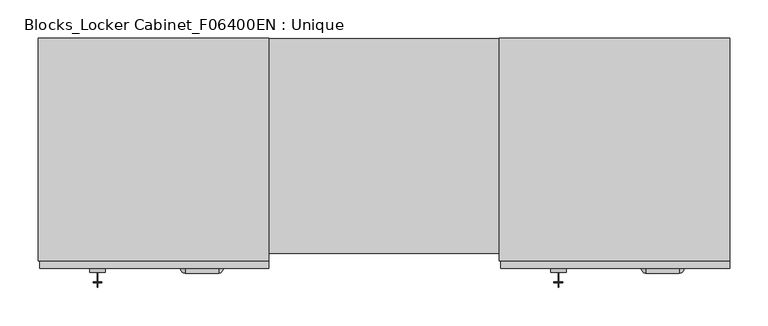
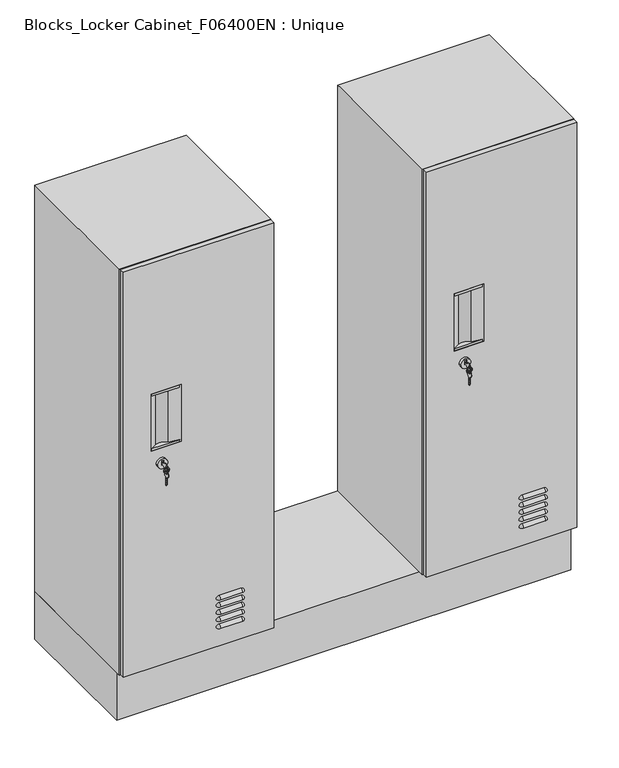
"""IFC4 building model written with IfcOpenShell, lengths in millimetres: furniture geometry, Blocks_Locker Cabinet_F06400EN : Unique."""

from ifc_helpers import new_model, si_unit, point, frame, frame_2d, origin, origin_with_axes, place, context, project, spatial, polyline, circle_curve, ellipse_curve, trimmed, segment, composite_curve, outline, extrude, faceted_brep, source, transform, mapped, element, save
from ifc_brep_helpers import plane_surface, cylinder_surface, revolved_surface, advanced_brep


def blocks_locker_cabinet_f06400en_unique_45afab01(model_context):
    return source(origin(), model_context, "Body", "SolidModel", [
        advanced_brep(
        [(217.0, -12.5, 525.0), (237.0, -12.5, 525.0), (228.8411805, -12.5, 532.0962926), (228.8411805, -12.5, 522.8618188), (225.1588195, -12.5, 522.8618188), (225.1588195, -12.5, 532.0962926), (217.0, -7.5, 525.0), (237.0, -7.5, 525.0), (217.0, -10.7450625, 525.0), (237.0, -10.7450625, 525.0), (228.8411805, -10.7450625, 532.0962926), (228.8411805, -10.7450625, 522.8618188), (225.1588195, -10.7450625, 522.8618188), (225.1588195, -10.7450625, 532.0962926)],
        [
            (0, 1, circle_curve(frame((227.0, -12.5, 525.0), z_axis=(0.0, -1.0, 0.0), x_axis=(1.0, 0.0, 0.0)), 10.0)),
            (1, 0, circle_curve(frame((227.0, -12.5, 525.0), z_axis=(0.0, -1.0, 0.0), x_axis=(1.0, 0.0, 0.0)), 10.0)),
            (2, 3),
            (3, 4),
            (4, 5),
            (5, 2),
            (6, 7, circle_curve(frame((227.0, -7.5, 525.0), z_axis=(0.0, 1.0, 0.0), x_axis=(1.0, 0.0, 0.0)), 10.0)),
            (7, 6, circle_curve(frame((227.0, -7.5, 525.0), z_axis=(0.0, 1.0, 0.0), x_axis=(1.0, 0.0, 0.0)), 10.0)),
            (0, 8),
            (8, 6),
            (7, 9),
            (9, 1),
            (2, 10),
            (10, 11),
            (11, 3),
            (11, 12),
            (12, 4),
            (12, 13),
            (13, 5),
            (13, 10),
        ],
        [
            plane_surface(frame((237.0, -12.5, 525.0), z_axis=(0.0, -1.0, 0.0), x_axis=(0.0, 0.0, 1.0))),
            plane_surface(frame((237.0, -7.5, 525.0), z_axis=(0.0, 1.0, 0.0), x_axis=(0.0, 0.0, -1.0))),
            cylinder_surface(frame((227.0, -7.5, 525.0), z_axis=(0.0, -1.0, 0.0), x_axis=(1.0, 0.0, 0.0)), 10.0),
            plane_surface(frame((228.8411805, -12.5, 532.0962926), z_axis=(-1.0, 0.0, 0.0), x_axis=(0.0, 1.0, 0.0))),
            plane_surface(frame((228.8411805, -12.5, 522.8618188), z_axis=(0.0, 0.0, 1.0), x_axis=(0.0, 1.0, 0.0))),
            plane_surface(frame((225.1588195, -12.5, 522.8618188), z_axis=(1.0, 0.0, 0.0), x_axis=(0.0, 1.0, 0.0))),
            plane_surface(frame((225.1588195, -12.5, 532.0962926), z_axis=(0.0, 0.0, -1.0), x_axis=(0.0, 1.0, 0.0))),
            plane_surface(frame((237.0, -10.7450625, 525.0), z_axis=(0.0, -1.0, 0.0), x_axis=(0.0, 0.0, 1.0))),
        ],
        [
            (0, [[1, 2], [3, 4, 5, 6]]),
            (1, [[7, 8]]),
            (2, [[-1, 9, 10, -8, 11, 12]]),
            (2, [[-2, -12, -11, -7, -10, -9]]),
            (3, [[-3, 13, 14, 15]]),
            (4, [[-4, -15, 16, 17]]),
            (5, [[-5, -17, 18, 19]]),
            (6, [[-6, -19, 20, -13]]),
            (7, [[-14, -20, -18, -16]]),
        ],
    ),
        extrude(outline(composite_curve([segment(trimmed(circle_curve(frame_2d((-23.0067332, 525.0)), 6.5414185), [point((-16.8246351, 522.8618188))], [point((-17.0336838, 527.6669902))], False, "CARTESIAN"), True, "CONTINUOUS"), segment(polyline([(-17.0336838, 527.6669902), (-10.7450625, 527.6669902), (-10.7450625, 522.8618188), (-12.0321832, 522.8618188)]), True, "CONTINUOUS"), segment(trimmed(circle_curve(frame_2d((-12.908516, 522.8618188)), 0.8763328), [point((-12.0321832, 522.8618188))], [point((-13.7848488, 522.8618188))], True, "CARTESIAN"), True, "CONTINUOUS"), segment(polyline([(-13.7848488, 522.8618188), (-16.8246351, 522.8618188)]), True, "CONTINUOUS")], self_intersect=False), holes=[composite_curve([segment(trimmed(circle_curve(frame_2d((-25.6281997, 525.0)), 1.688217), [point((-27.3164167, 525.0))], [point((-23.9399827, 525.0))], True, "CARTESIAN"), True, "CONTINUOUS"), segment(trimmed(circle_curve(frame_2d((-25.6281997, 525.0)), 1.688217), [point((-23.9399827, 525.0))], [point((-27.3164167, 525.0))], True, "CARTESIAN"), True, "CONTINUOUS")], self_intersect=False)]), frame((226.5956922, 0.0, 0.0), z_axis=(1.0, 0.0, 0.0), x_axis=(0.0, 1.0, 0.0)), (0.0, 0.0, 1.0), 0.9157402),
        extrude(outline(composite_curve([segment(trimmed(circle_curve(frame_2d((-25.6743188, 510.9839856)), 6.5414185), [point((-27.8125, 504.8018875))], [point((-24.2573286, 504.5978839))], False, "CARTESIAN"), True, "CONTINUOUS"), segment(polyline([(-24.2573286, 504.5978839), (-24.2573286, 487.7095301), (-25.9613419, 487.7095301), (-27.8125, 490.3532579), (-27.8125, 492.0094356)]), True, "CONTINUOUS"), segment(trimmed(circle_curve(frame_2d((-27.8125, 492.8857684)), 0.8763328), [point((-27.8125, 492.0094356))], [point((-27.8125, 493.7621012))], True, "CARTESIAN"), True, "CONTINUOUS"), segment(polyline([(-27.8125, 493.7621012), (-27.8125, 496.0094356)]), True, "CONTINUOUS"), segment(trimmed(circle_curve(frame_2d((-27.8125, 496.8857684)), 0.8763328), [point((-27.8125, 496.0094356))], [point((-27.8125, 497.7621012))], True, "CARTESIAN"), True, "CONTINUOUS"), segment(polyline([(-27.8125, 497.7621012), (-27.8125, 500.0094356)]), True, "CONTINUOUS"), segment(trimmed(circle_curve(frame_2d((-27.8125, 500.8857684)), 0.8763328), [point((-27.8125, 500.0094356))], [point((-27.8125, 501.7621012))], True, "CARTESIAN"), True, "CONTINUOUS"), segment(polyline([(-27.8125, 501.7621012), (-27.8125, 504.8018875)]), True, "CONTINUOUS")], self_intersect=False), holes=[composite_curve([segment(trimmed(circle_curve(frame_2d((-25.6743188, 513.6054521)), 1.688217), [point((-25.6743188, 515.2936691))], [point((-25.6743188, 511.9172351))], True, "CARTESIAN"), True, "CONTINUOUS"), segment(trimmed(circle_curve(frame_2d((-25.6743188, 513.6054521)), 1.688217), [point((-25.6743188, 511.9172351))], [point((-25.6743188, 515.2936691))], True, "CARTESIAN"), True, "CONTINUOUS")], self_intersect=False)]), frame((226.5956922, 0.0, 0.0), z_axis=(1.0, 0.0, 0.0), x_axis=(0.0, 1.0, 0.0)), (0.0, 0.0, 1.0), 0.9157402),
        advanced_brep(
        [(231.2, -25.663019, 519.4000012), (222.8, -25.663019, 519.4000012), (221.2, -25.663019, 519.4000012), (232.8, -25.663019, 519.4000012)],
        [
            (0, 1, circle_curve(frame((227.0, -25.663019, 519.4000012), z_axis=(0.0, 1.0, 0.0), x_axis=(-1.0, 0.0, 0.0)), 4.2)),
            (1, 2, circle_curve(frame((222.0, -25.663019, 519.4000012), z_axis=(0.0, 0.0, -1.0), x_axis=(1.0, 0.0, 0.0)), 0.8)),
            (2, 3, circle_curve(frame((227.0, -25.663019, 519.4000012), z_axis=(0.0, -1.0, 0.0), x_axis=(-1.0, 0.0, 0.0)), 5.8)),
            (3, 0, circle_curve(frame((232.0, -25.663019, 519.4000012), z_axis=(0.0, 0.0, -1.0), x_axis=(-1.0, 0.0, 0.0)), 0.8)),
            (2, 1, circle_curve(frame((222.0, -25.663019, 519.4000012), z_axis=(0.0, 0.0, -1.0), x_axis=(1.0, 0.0, 0.0)), 0.8)),
            (0, 3, circle_curve(frame((232.0, -25.663019, 519.4000012), z_axis=(0.0, 0.0, -1.0), x_axis=(-1.0, 0.0, 0.0)), 0.8)),
            (1, 0, circle_curve(frame((227.0, -25.663019, 519.4000012), z_axis=(0.0, 1.0, 0.0), x_axis=(1.0, 0.0, 0.0)), 4.2)),
            (3, 2, circle_curve(frame((227.0, -25.663019, 519.4000012), z_axis=(0.0, -1.0, 0.0), x_axis=(1.0, 0.0, 0.0)), 5.8)),
        ],
        [
            revolved_surface(trimmed(ellipse_curve(frame((222.0, -25.663019, 519.4000012), z_axis=(0.0, 0.0, 1.0), x_axis=(1.0, 0.0, 0.0)), 0.8, 0.8), [point((221.2, -25.663019, 519.4000012))], [point((222.8, -25.663019, 519.4000012))], True, "CARTESIAN"), (227.0, 2.5, 519.4000012), (0.0, -1.0, 0.0)),
            revolved_surface(trimmed(ellipse_curve(frame((222.0, -25.663019, 519.4000012), z_axis=(0.0, 0.0, 1.0), x_axis=(1.0, 0.0, 0.0)), 0.8, 0.8), [point((222.8, -25.663019, 519.4000012))], [point((221.2, -25.663019, 519.4000012))], True, "CARTESIAN"), (227.0, 2.5, 519.4000012), (0.0, -1.0, 0.0)),
            revolved_surface(trimmed(ellipse_curve(frame((232.0, -25.663019, 519.4000012), z_axis=(0.0, 0.0, -1.0), x_axis=(-1.0, 0.0, 0.0)), 0.8, 0.8), [point((232.8, -25.663019, 519.4000012))], [point((231.2, -25.663019, 519.4000012))], True, "CARTESIAN"), (227.0, 2.5, 519.4000012), (0.0, -1.0, 0.0)),
            revolved_surface(trimmed(ellipse_curve(frame((232.0, -25.663019, 519.4000012), z_axis=(0.0, 0.0, -1.0), x_axis=(-1.0, 0.0, 0.0)), 0.8, 0.8), [point((231.2, -25.663019, 519.4000012))], [point((232.8, -25.663019, 519.4000012))], True, "CARTESIAN"), (227.0, 2.5, 519.4000012), (0.0, -1.0, 0.0)),
        ],
        [
            (0, [[1, 2, 3, 4]]),
            (1, [[-3, 5, -1, 6]]),
            (2, [[7, -4, 8, -2]]),
            (3, [[-8, -6, -7, -5]]),
        ],
    ),
        advanced_brep(
        [(152.0, -7.5, 949.0), (450.0, -7.5, 949.0), (450.0, 2.5, 949.0), (152.0, 2.5, 949.0), (152.0, -7.5, 101.0), (152.0, 2.5, 101.0), (450.0, 2.5, 101.0), (450.0, -7.5, 101.0), (207.0, -7.5, 675.0), (266.2109264, -7.5, 675.0), (266.2109264, -7.5, 555.0), (207.0, -7.5, 555.0), (219.3473099, -0.3712773, 675.0), (242.7894451, -3.975278, 675.0), (219.3473099, -0.3712773, 555.0), (242.7894451, -3.975278, 555.0)],
        [
            (0, 1),
            (1, 2),
            (2, 3),
            (3, 0),
            (4, 5),
            (5, 6),
            (6, 7),
            (7, 4),
            (0, 4),
            (7, 1),
            (8, 9),
            (9, 10),
            (10, 11),
            (11, 8),
            (6, 2),
            (5, 3),
            (12, 13, circle_curve(frame((228.8223477, -16.7825242, 675.0), z_axis=(0.0, 0.0, -1.0), x_axis=(0.0, -1.0, 0.0)), 18.9500756)),
            (13, 9),
            (8, 12),
            (14, 11),
            (10, 15),
            (15, 14, circle_curve(frame((228.8223477, -16.7825242, 555.0), z_axis=(0.0, 0.0, 1.0), x_axis=(0.0, -1.0, 0.0)), 18.9500756)),
            (14, 12),
            (13, 15),
        ],
        [
            plane_surface(frame((450.0, -7.5, 949.0), z_axis=(0.0, 0.0, 1.0), x_axis=(1.0, 0.0, 0.0))),
            plane_surface(frame((450.0, -7.5, 101.0), z_axis=(0.0, 0.0, -1.0), x_axis=(-1.0, 0.0, 0.0))),
            plane_surface(frame((152.0, -7.5, 949.0), z_axis=(0.0, -1.0, 0.0), x_axis=(0.0, 0.0, -1.0))),
            plane_surface(frame((450.0, -7.5, 949.0), z_axis=(1.0, 0.0, 0.0), x_axis=(0.0, 0.0, -1.0))),
            plane_surface(frame((450.0, 2.5, 949.0), z_axis=(0.0, 1.0, 0.0), x_axis=(0.0, 0.0, -1.0))),
            plane_surface(frame((152.0, 2.5, 949.0), z_axis=(-1.0, 0.0, 0.0), x_axis=(0.0, 0.0, -1.0))),
            plane_surface(frame((207.0, -7.5, 675.0), z_axis=(0.0, 0.0, -1.0), x_axis=(-0.866025403784437, -0.5000000000000028, 0.0))),
            plane_surface(frame((207.0, -7.5, 555.0), z_axis=(0.0, 0.0, 1.0), x_axis=(0.866025403784437, 0.5000000000000028, 0.0))),
            plane_surface(frame((219.3473099, -0.3712773, 675.0), z_axis=(0.5000000000000028, -0.866025403784437, 0.0), x_axis=(0.0, 0.0, -1.0))),
            plane_surface(frame((266.2109264, -7.5, 675.0), z_axis=(-0.14881527984319862, -0.9888650122666847, 0.0), x_axis=(0.0, 0.0, -1.0))),
            revolved_surface(polyline([(228.8223477, -35.7325998, 675.0), (228.8223477, -35.7325998, 555.0)]), (228.8223477, -16.7825242, 555.0), (0.0, 0.0, 1.0)),
        ],
        [
            (0, [[1, 2, 3, 4]]),
            (1, [[5, 6, 7, 8]]),
            (2, [[-1, 9, -8, 10], [11, 12, 13, 14]]),
            (3, [[-2, -10, -7, 15]]),
            (4, [[-3, -15, -6, 16]]),
            (5, [[-4, -16, -5, -9]]),
            (6, [[17, 18, -11, 19]]),
            (7, [[20, -13, 21, 22]]),
            (8, [[-19, -14, -20, 23]]),
            (9, [[-18, 24, -21, -12]]),
            (10, [[-17, -23, -22, -24]]),
        ],
    ),
        advanced_brep(
        [(335.0, -7.5, 141.0), (341.0, -7.5, 147.0), (384.5189667, -7.5, 147.0), (390.5189667, -7.5, 141.0), (384.5189667, -13.5, 141.0), (341.0, -13.5, 141.0)],
        [
            (0, 1, circle_curve(frame((341.0, -7.5, 141.0), z_axis=(0.0, 1.0, 0.0), x_axis=(1.0, 0.0, 0.0)), 6.0)),
            (1, 2),
            (2, 3, circle_curve(frame((384.5189667, -7.5, 141.0), z_axis=(0.0, 1.0, 0.0), x_axis=(1.0, 0.0, 0.0)), 6.0)),
            (3, 0),
            (3, 4, circle_curve(frame((384.5189667, -7.5, 141.0), z_axis=(0.0, 0.0, -1.0), x_axis=(1.0, 0.0, 0.0)), 6.0)),
            (4, 5),
            (5, 0, circle_curve(frame((341.0, -7.5, 141.0), z_axis=(0.0, 0.0, -1.0), x_axis=(1.0, 0.0, 0.0)), 6.0)),
            (5, 1, circle_curve(frame((341.0, -7.5, 141.0), z_axis=(-1.0, 0.0, 0.0), x_axis=(0.0, 0.0, 1.0)), 6.0)),
            (4, 2, circle_curve(frame((384.5189667, -7.5, 141.0), z_axis=(-1.0, 0.0, 0.0), x_axis=(0.0, 0.0, 1.0)), 6.0)),
        ],
        [
            plane_surface(frame((385.0, -7.5, 141.0), z_axis=(0.0, 1.0, 0.0), x_axis=(0.0, 0.0, 1.0))),
            plane_surface(frame((385.0, -7.5, 141.0), z_axis=(0.0, 0.0, -1.0), x_axis=(0.0, -1.0, 0.0))),
            revolved_surface(trimmed(ellipse_curve(frame((341.0, -7.5, 141.0), z_axis=(0.0, 1.0, 0.0), x_axis=(1.0, 0.0, 0.0)), 6.0, 6.0), [point((335.0, -7.5, 141.0))], [point((341.0, -7.5, 147.0))], True, "CARTESIAN"), (385.0, -7.5, 141.0), (1.0, 0.0, 0.0)),
            cylinder_surface(frame((385.0, -7.5, 141.0), z_axis=(1.0, 0.0, 0.0), x_axis=(0.0, 0.0, 1.0)), 6.0),
            revolved_surface(trimmed(ellipse_curve(frame((384.5189667, -7.5, 141.0), z_axis=(0.0, 1.0, 0.0), x_axis=(1.0, 0.0, 0.0)), 6.0, 6.0), [point((384.5189667, -7.5, 147.0))], [point((390.5189667, -7.5, 141.0))], True, "CARTESIAN"), (385.0, -7.5, 141.0), (1.0, 0.0, 0.0)),
        ],
        [
            (0, [[1, 2, 3, 4]]),
            (1, [[5, 6, 7, -4]]),
            (2, [[8, -1, -7]]),
            (3, [[9, -2, -8, -6]]),
            (4, [[-3, -9, -5]]),
        ],
    ),
        advanced_brep(
        [(335.0, -7.5, 156.0), (341.0, -7.5, 162.0), (384.5189667, -7.5, 162.0), (390.5189667, -7.5, 156.0), (384.5189667, -13.5, 156.0), (341.0, -13.5, 156.0)],
        [
            (0, 1, circle_curve(frame((341.0, -7.5, 156.0), z_axis=(0.0, 1.0, 0.0), x_axis=(1.0, 0.0, 0.0)), 6.0)),
            (1, 2),
            (2, 3, circle_curve(frame((384.5189667, -7.5, 156.0), z_axis=(0.0, 1.0, 0.0), x_axis=(1.0, 0.0, 0.0)), 6.0)),
            (3, 0),
            (3, 4, circle_curve(frame((384.5189667, -7.5, 156.0), z_axis=(0.0, 0.0, -1.0), x_axis=(1.0, 0.0, 0.0)), 6.0)),
            (4, 5),
            (5, 0, circle_curve(frame((341.0, -7.5, 156.0), z_axis=(0.0, 0.0, -1.0), x_axis=(1.0, 0.0, 0.0)), 6.0)),
            (5, 1, circle_curve(frame((341.0, -7.5, 156.0), z_axis=(-1.0, 0.0, 0.0), x_axis=(0.0, 0.0, 1.0)), 6.0)),
            (4, 2, circle_curve(frame((384.5189667, -7.5, 156.0), z_axis=(-1.0, 0.0, 0.0), x_axis=(0.0, 0.0, 1.0)), 6.0)),
        ],
        [
            plane_surface(frame((385.0, -7.5, 156.0), z_axis=(0.0, 1.0, 0.0), x_axis=(0.0, 0.0, 1.0))),
            plane_surface(frame((385.0, -7.5, 156.0), z_axis=(0.0, 0.0, -1.0), x_axis=(0.0, -1.0, 0.0))),
            revolved_surface(trimmed(ellipse_curve(frame((341.0, -7.5, 156.0), z_axis=(0.0, 1.0, 0.0), x_axis=(1.0, 0.0, 0.0)), 6.0, 6.0), [point((335.0, -7.5, 156.0))], [point((341.0, -7.5, 162.0))], True, "CARTESIAN"), (385.0, -7.5, 156.0), (1.0, 0.0, 0.0)),
            cylinder_surface(frame((385.0, -7.5, 156.0), z_axis=(1.0, 0.0, 0.0), x_axis=(0.0, 0.0, 1.0)), 6.0),
            revolved_surface(trimmed(ellipse_curve(frame((384.5189667, -7.5, 156.0), z_axis=(0.0, 1.0, 0.0), x_axis=(1.0, 0.0, 0.0)), 6.0, 6.0), [point((384.5189667, -7.5, 162.0))], [point((390.5189667, -7.5, 156.0))], True, "CARTESIAN"), (385.0, -7.5, 156.0), (1.0, 0.0, 0.0)),
        ],
        [
            (0, [[1, 2, 3, 4]]),
            (1, [[5, 6, 7, -4]]),
            (2, [[8, -1, -7]]),
            (3, [[9, -2, -8, -6]]),
            (4, [[-3, -9, -5]]),
        ],
    ),
        advanced_brep(
        [(335.0, -7.5, 171.0), (341.0, -7.5, 177.0), (384.5189667, -7.5, 177.0), (390.5189667, -7.5, 171.0), (384.5189667, -13.5, 171.0), (341.0, -13.5, 171.0)],
        [
            (0, 1, circle_curve(frame((341.0, -7.5, 171.0), z_axis=(0.0, 1.0, 0.0), x_axis=(1.0, 0.0, 0.0)), 6.0)),
            (1, 2),
            (2, 3, circle_curve(frame((384.5189667, -7.5, 171.0), z_axis=(0.0, 1.0, 0.0), x_axis=(1.0, 0.0, 0.0)), 6.0)),
            (3, 0),
            (3, 4, circle_curve(frame((384.5189667, -7.5, 171.0), z_axis=(0.0, 0.0, -1.0), x_axis=(1.0, 0.0, 0.0)), 6.0)),
            (4, 5),
            (5, 0, circle_curve(frame((341.0, -7.5, 171.0), z_axis=(0.0, 0.0, -1.0), x_axis=(1.0, 0.0, 0.0)), 6.0)),
            (5, 1, circle_curve(frame((341.0, -7.5, 171.0), z_axis=(-1.0, 0.0, 0.0), x_axis=(0.0, 0.0, 1.0)), 6.0)),
            (4, 2, circle_curve(frame((384.5189667, -7.5, 171.0), z_axis=(-1.0, 0.0, 0.0), x_axis=(0.0, 0.0, 1.0)), 6.0)),
        ],
        [
            plane_surface(frame((385.0, -7.5, 171.0), z_axis=(0.0, 1.0, 0.0), x_axis=(0.0, 0.0, 1.0))),
            plane_surface(frame((385.0, -7.5, 171.0), z_axis=(0.0, 0.0, -1.0), x_axis=(0.0, -1.0, 0.0))),
            revolved_surface(trimmed(ellipse_curve(frame((341.0, -7.5, 171.0), z_axis=(0.0, 1.0, 0.0), x_axis=(1.0, 0.0, 0.0)), 6.0, 6.0), [point((335.0, -7.5, 171.0))], [point((341.0, -7.5, 177.0))], True, "CARTESIAN"), (385.0, -7.5, 171.0), (1.0, 0.0, 0.0)),
            cylinder_surface(frame((385.0, -7.5, 171.0), z_axis=(1.0, 0.0, 0.0), x_axis=(0.0, 0.0, 1.0)), 6.0),
            revolved_surface(trimmed(ellipse_curve(frame((384.5189667, -7.5, 171.0), z_axis=(0.0, 1.0, 0.0), x_axis=(1.0, 0.0, 0.0)), 6.0, 6.0), [point((384.5189667, -7.5, 177.0))], [point((390.5189667, -7.5, 171.0))], True, "CARTESIAN"), (385.0, -7.5, 171.0), (1.0, 0.0, 0.0)),
        ],
        [
            (0, [[1, 2, 3, 4]]),
            (1, [[5, 6, 7, -4]]),
            (2, [[8, -1, -7]]),
            (3, [[9, -2, -8, -6]]),
            (4, [[-3, -9, -5]]),
        ],
    ),
        advanced_brep(
        [(335.0, -7.5, 186.0), (341.0, -7.5, 192.0), (384.5189667, -7.5, 192.0), (390.5189667, -7.5, 186.0), (384.5189667, -13.5, 186.0), (341.0, -13.5, 186.0)],
        [
            (0, 1, circle_curve(frame((341.0, -7.5, 186.0), z_axis=(0.0, 1.0, 0.0), x_axis=(1.0, 0.0, 0.0)), 6.0)),
            (1, 2),
            (2, 3, circle_curve(frame((384.5189667, -7.5, 186.0), z_axis=(0.0, 1.0, 0.0), x_axis=(1.0, 0.0, 0.0)), 6.0)),
            (3, 0),
            (3, 4, circle_curve(frame((384.5189667, -7.5, 186.0), z_axis=(0.0, 0.0, -1.0), x_axis=(1.0, 0.0, 0.0)), 6.0)),
            (4, 5),
            (5, 0, circle_curve(frame((341.0, -7.5, 186.0), z_axis=(0.0, 0.0, -1.0), x_axis=(1.0, 0.0, 0.0)), 6.0)),
            (5, 1, circle_curve(frame((341.0, -7.5, 186.0), z_axis=(-1.0, 0.0, 0.0), x_axis=(0.0, 0.0, 1.0)), 6.0)),
            (4, 2, circle_curve(frame((384.5189667, -7.5, 186.0), z_axis=(-1.0, 0.0, 0.0), x_axis=(0.0, 0.0, 1.0)), 6.0)),
        ],
        [
            plane_surface(frame((385.0, -7.5, 186.0), z_axis=(0.0, 1.0, 0.0), x_axis=(0.0, 0.0, 1.0))),
            plane_surface(frame((385.0, -7.5, 186.0), z_axis=(0.0, 0.0, -1.0), x_axis=(0.0, -1.0, 0.0))),
            revolved_surface(trimmed(ellipse_curve(frame((341.0, -7.5, 186.0), z_axis=(0.0, 1.0, 0.0), x_axis=(1.0, 0.0, 0.0)), 6.0, 6.0), [point((335.0, -7.5, 186.0))], [point((341.0, -7.5, 192.0))], True, "CARTESIAN"), (385.0, -7.5, 186.0), (1.0, 0.0, 0.0)),
            cylinder_surface(frame((385.0, -7.5, 186.0), z_axis=(1.0, 0.0, 0.0), x_axis=(0.0, 0.0, 1.0)), 6.0),
            revolved_surface(trimmed(ellipse_curve(frame((384.5189667, -7.5, 186.0), z_axis=(0.0, 1.0, 0.0), x_axis=(1.0, 0.0, 0.0)), 6.0, 6.0), [point((384.5189667, -7.5, 192.0))], [point((390.5189667, -7.5, 186.0))], True, "CARTESIAN"), (385.0, -7.5, 186.0), (1.0, 0.0, 0.0)),
        ],
        [
            (0, [[1, 2, 3, 4]]),
            (1, [[5, 6, 7, -4]]),
            (2, [[8, -1, -7]]),
            (3, [[9, -2, -8, -6]]),
            (4, [[-3, -9, -5]]),
        ],
    ),
        advanced_brep(
        [(335.0, -7.5, 201.0), (341.0, -7.5, 207.0), (384.5189667, -7.5, 207.0), (390.5189667, -7.5, 201.0), (384.5189667, -13.5, 201.0), (341.0, -13.5, 201.0)],
        [
            (0, 1, circle_curve(frame((341.0, -7.5, 201.0), z_axis=(0.0, 1.0, 0.0), x_axis=(1.0, 0.0, 0.0)), 6.0)),
            (1, 2),
            (2, 3, circle_curve(frame((384.5189667, -7.5, 201.0), z_axis=(0.0, 1.0, 0.0), x_axis=(1.0, 0.0, 0.0)), 6.0)),
            (3, 0),
            (3, 4, circle_curve(frame((384.5189667, -7.5, 201.0), z_axis=(0.0, 0.0, -1.0), x_axis=(1.0, 0.0, 0.0)), 6.0)),
            (4, 5),
            (5, 0, circle_curve(frame((341.0, -7.5, 201.0), z_axis=(0.0, 0.0, -1.0), x_axis=(1.0, 0.0, 0.0)), 6.0)),
            (5, 1, circle_curve(frame((341.0, -7.5, 201.0), z_axis=(-1.0, 0.0, 0.0), x_axis=(0.0, 0.0, 1.0)), 6.0)),
            (4, 2, circle_curve(frame((384.5189667, -7.5, 201.0), z_axis=(-1.0, 0.0, 0.0), x_axis=(0.0, 0.0, 1.0)), 6.0)),
        ],
        [
            plane_surface(frame((385.0, -7.5, 201.0), z_axis=(0.0, 1.0, 0.0), x_axis=(0.0, 0.0, 1.0))),
            plane_surface(frame((385.0, -7.5, 201.0), z_axis=(0.0, 0.0, -1.0), x_axis=(0.0, -1.0, 0.0))),
            revolved_surface(trimmed(ellipse_curve(frame((341.0, -7.5, 201.0), z_axis=(0.0, 1.0, 0.0), x_axis=(1.0, 0.0, 0.0)), 6.0, 6.0), [point((335.0, -7.5, 201.0))], [point((341.0, -7.5, 207.0))], True, "CARTESIAN"), (385.0, -7.5, 201.0), (1.0, 0.0, 0.0)),
            cylinder_surface(frame((385.0, -7.5, 201.0), z_axis=(1.0, 0.0, 0.0), x_axis=(0.0, 0.0, 1.0)), 6.0),
            revolved_surface(trimmed(ellipse_curve(frame((384.5189667, -7.5, 201.0), z_axis=(0.0, 1.0, 0.0), x_axis=(1.0, 0.0, 0.0)), 6.0, 6.0), [point((384.5189667, -7.5, 207.0))], [point((390.5189667, -7.5, 201.0))], True, "CARTESIAN"), (385.0, -7.5, 201.0), (1.0, 0.0, 0.0)),
        ],
        [
            (0, [[1, 2, 3, 4]]),
            (1, [[5, 6, 7, -4]]),
            (2, [[8, -1, -7]]),
            (3, [[9, -2, -8, -6]]),
            (4, [[-3, -9, -5]]),
        ],
    ),
        extrude(outline(composite_curve([segment(trimmed(circle_curve(frame_2d((228.8223477, -16.7825242)), 18.9500756), [point((219.3473099, -0.3712773))], [point((242.7894451, -3.975278))], False, "CARTESIAN"), True, "CONTINUOUS"), segment(polyline([(242.7894451, -3.975278), (266.2109264, -7.5), (207.0, -7.5), (219.3473099, -0.3712773)]), True, "CONTINUOUS")], self_intersect=False)), frame((0.0, 0.0, 555.0), z_axis=(0.0, 0.0, 1.0), x_axis=(1.0, 0.0, 0.0)), (0.0, 0.0, 1.0), 5.0),
        extrude(outline(composite_curve([segment(trimmed(circle_curve(frame_2d((228.8223477, -16.7825242)), 18.9500756), [point((219.3473099, -0.3712773))], [point((242.7894451, -3.975278))], False, "CARTESIAN"), True, "CONTINUOUS"), segment(polyline([(242.7894451, -3.975278), (266.2109264, -7.5), (207.0, -7.5), (219.3473099, -0.3712773)]), True, "CONTINUOUS")], self_intersect=False)), frame((0.0, 0.0, 670.0), z_axis=(0.0, 0.0, 1.0), x_axis=(1.0, 0.0, 0.0)), (0.0, 0.0, 1.0), 5.0),
        faceted_brep([(450.0, 2.5, 950.0), (150.0, 2.5, 950.0), (150.0, 2.5, 100.0), (450.0, 2.5, 100.0), (440.0, 2.5, 940.0), (440.0, 2.5, 110.0), (160.0, 2.5, 110.0), (160.0, 2.5, 940.0), (450.0, 292.5, 950.0), (450.0, 292.5, 100.0), (150.0, 292.5, 100.0), (150.0, 292.5, 950.0), (450.0, 282.5, 950.0), (150.0, 282.5, 950.0), (150.0, 282.5, 100.0), (450.0, 282.5, 100.0), (440.0, 282.5, 940.0), (440.0, 282.5, 110.0), (160.0, 282.5, 110.0), (160.0, 282.5, 940.0)], [[[0, 1, 2, 3], [4, 5, 6, 7]], [[8, 9, 10, 11]], [[1, 0, 12, 8, 11, 13]], [[2, 1, 13, 11, 10, 14]], [[3, 2, 14, 10, 9, 15]], [[0, 3, 15, 9, 8, 12]], [[5, 4, 16, 17]], [[6, 5, 17, 18]], [[7, 6, 18, 19]], [[4, 7, 19, 16]], [[17, 16, 19, 18]]]),
        advanced_brep(
        [(-383.0, -12.5, 525.0), (-363.0, -12.5, 525.0), (-371.1588195, -12.5, 532.0962926), (-371.1588195, -12.5, 522.8618188), (-374.8411805, -12.5, 522.8618188), (-374.8411805, -12.5, 532.0962926), (-383.0, -7.5, 525.0), (-363.0, -7.5, 525.0), (-383.0, -10.7450625, 525.0), (-363.0, -10.7450625, 525.0), (-371.1588195, -10.7450625, 532.0962926), (-371.1588195, -10.7450625, 522.8618188), (-374.8411805, -10.7450625, 522.8618188), (-374.8411805, -10.7450625, 532.0962926)],
        [
            (0, 1, circle_curve(frame((-373.0, -12.5, 525.0), z_axis=(0.0, -1.0, 0.0), x_axis=(1.0, 0.0, 0.0)), 10.0)),
            (1, 0, circle_curve(frame((-373.0, -12.5, 525.0), z_axis=(0.0, -1.0, 0.0), x_axis=(1.0, 0.0, 0.0)), 10.0)),
            (2, 3),
            (3, 4),
            (4, 5),
            (5, 2),
            (6, 7, circle_curve(frame((-373.0, -7.5, 525.0), z_axis=(0.0, 1.0, 0.0), x_axis=(1.0, 0.0, 0.0)), 10.0)),
            (7, 6, circle_curve(frame((-373.0, -7.5, 525.0), z_axis=(0.0, 1.0, 0.0), x_axis=(1.0, 0.0, 0.0)), 10.0)),
            (0, 8),
            (8, 6),
            (7, 9),
            (9, 1),
            (2, 10),
            (10, 11),
            (11, 3),
            (11, 12),
            (12, 4),
            (12, 13),
            (13, 5),
            (13, 10),
        ],
        [
            plane_surface(frame((-363.0, -12.5, 525.0), z_axis=(0.0, -1.0, 0.0), x_axis=(0.0, 0.0, 1.0))),
            plane_surface(frame((-363.0, -7.5, 525.0), z_axis=(0.0, 1.0, 0.0), x_axis=(0.0, 0.0, -1.0))),
            cylinder_surface(frame((-373.0, -7.5, 525.0), z_axis=(0.0, -1.0, 0.0), x_axis=(1.0, 0.0, 0.0)), 10.0),
            plane_surface(frame((-371.1588195, -12.5, 532.0962926), z_axis=(-1.0, 0.0, 0.0), x_axis=(0.0, 1.0, 0.0))),
            plane_surface(frame((-371.1588195, -12.5, 522.8618188), z_axis=(0.0, 0.0, 1.0), x_axis=(0.0, 1.0, 0.0))),
            plane_surface(frame((-374.8411805, -12.5, 522.8618188), z_axis=(1.0, 0.0, 0.0), x_axis=(0.0, 1.0, 0.0))),
            plane_surface(frame((-374.8411805, -12.5, 532.0962926), z_axis=(0.0, 0.0, -1.0), x_axis=(0.0, 1.0, 0.0))),
            plane_surface(frame((-363.0, -10.7450625, 525.0), z_axis=(0.0, -1.0, 0.0), x_axis=(0.0, 0.0, 1.0))),
        ],
        [
            (0, [[1, 2], [3, 4, 5, 6]]),
            (1, [[7, 8]]),
            (2, [[-1, 9, 10, -8, 11, 12]]),
            (2, [[-2, -12, -11, -7, -10, -9]]),
            (3, [[-3, 13, 14, 15]]),
            (4, [[-4, -15, 16, 17]]),
            (5, [[-5, -17, 18, 19]]),
            (6, [[-6, -19, 20, -13]]),
            (7, [[-14, -20, -18, -16]]),
        ],
    ),
        extrude(outline(composite_curve([segment(trimmed(circle_curve(frame_2d((-23.0067332, 525.0)), 6.5414185), [point((-16.8246351, 522.8618188))], [point((-17.0336838, 527.6669902))], False, "CARTESIAN"), True, "CONTINUOUS"), segment(polyline([(-17.0336838, 527.6669902), (-10.7450625, 527.6669902), (-10.7450625, 522.8618188), (-12.0321832, 522.8618188)]), True, "CONTINUOUS"), segment(trimmed(circle_curve(frame_2d((-12.908516, 522.8618188)), 0.8763328), [point((-12.0321832, 522.8618188))], [point((-13.7848488, 522.8618188))], True, "CARTESIAN"), True, "CONTINUOUS"), segment(polyline([(-13.7848488, 522.8618188), (-16.8246351, 522.8618188)]), True, "CONTINUOUS")], self_intersect=False), holes=[composite_curve([segment(trimmed(circle_curve(frame_2d((-25.6281997, 525.0)), 1.688217), [point((-27.3164167, 525.0))], [point((-23.9399827, 525.0))], True, "CARTESIAN"), True, "CONTINUOUS"), segment(trimmed(circle_curve(frame_2d((-25.6281997, 525.0)), 1.688217), [point((-23.9399827, 525.0))], [point((-27.3164167, 525.0))], True, "CARTESIAN"), True, "CONTINUOUS")], self_intersect=False)]), frame((-373.4043078, 0.0, 0.0), z_axis=(1.0, 0.0, 0.0), x_axis=(0.0, 1.0, 0.0)), (0.0, 0.0, 1.0), 0.9157402),
        extrude(outline(composite_curve([segment(trimmed(circle_curve(frame_2d((-25.6743188, 510.9839856)), 6.5414185), [point((-27.8125, 504.8018875))], [point((-24.2573286, 504.5978839))], False, "CARTESIAN"), True, "CONTINUOUS"), segment(polyline([(-24.2573286, 504.5978839), (-24.2573286, 487.7095301), (-25.9613419, 487.7095301), (-27.8125, 490.3532579), (-27.8125, 492.0094356)]), True, "CONTINUOUS"), segment(trimmed(circle_curve(frame_2d((-27.8125, 492.8857684)), 0.8763328), [point((-27.8125, 492.0094356))], [point((-27.8125, 493.7621012))], True, "CARTESIAN"), True, "CONTINUOUS"), segment(polyline([(-27.8125, 493.7621012), (-27.8125, 496.0094356)]), True, "CONTINUOUS"), segment(trimmed(circle_curve(frame_2d((-27.8125, 496.8857684)), 0.8763328), [point((-27.8125, 496.0094356))], [point((-27.8125, 497.7621012))], True, "CARTESIAN"), True, "CONTINUOUS"), segment(polyline([(-27.8125, 497.7621012), (-27.8125, 500.0094356)]), True, "CONTINUOUS"), segment(trimmed(circle_curve(frame_2d((-27.8125, 500.8857684)), 0.8763328), [point((-27.8125, 500.0094356))], [point((-27.8125, 501.7621012))], True, "CARTESIAN"), True, "CONTINUOUS"), segment(polyline([(-27.8125, 501.7621012), (-27.8125, 504.8018875)]), True, "CONTINUOUS")], self_intersect=False), holes=[composite_curve([segment(trimmed(circle_curve(frame_2d((-25.6743188, 513.6054521)), 1.688217), [point((-25.6743188, 515.2936691))], [point((-25.6743188, 511.9172351))], True, "CARTESIAN"), True, "CONTINUOUS"), segment(trimmed(circle_curve(frame_2d((-25.6743188, 513.6054521)), 1.688217), [point((-25.6743188, 511.9172351))], [point((-25.6743188, 515.2936691))], True, "CARTESIAN"), True, "CONTINUOUS")], self_intersect=False)]), frame((-373.4043078, 0.0, 0.0), z_axis=(1.0, 0.0, 0.0), x_axis=(0.0, 1.0, 0.0)), (0.0, 0.0, 1.0), 0.9157402),
        advanced_brep(
        [(-368.8, -25.663019, 519.4000012), (-377.2, -25.663019, 519.4000012), (-378.8, -25.663019, 519.4000012), (-367.2, -25.663019, 519.4000012)],
        [
            (0, 1, circle_curve(frame((-373.0, -25.663019, 519.4000012), z_axis=(0.0, 1.0, 0.0), x_axis=(-1.0, 0.0, 0.0)), 4.2)),
            (1, 2, circle_curve(frame((-378.0, -25.663019, 519.4000012), z_axis=(0.0, 0.0, -1.0), x_axis=(1.0, 0.0, 0.0)), 0.8)),
            (2, 3, circle_curve(frame((-373.0, -25.663019, 519.4000012), z_axis=(0.0, -1.0, 0.0), x_axis=(-1.0, 0.0, 0.0)), 5.8)),
            (3, 0, circle_curve(frame((-368.0, -25.663019, 519.4000012), z_axis=(0.0, 0.0, -1.0), x_axis=(-1.0, 0.0, 0.0)), 0.8)),
            (2, 1, circle_curve(frame((-378.0, -25.663019, 519.4000012), z_axis=(0.0, 0.0, -1.0), x_axis=(1.0, 0.0, 0.0)), 0.8)),
            (0, 3, circle_curve(frame((-368.0, -25.663019, 519.4000012), z_axis=(0.0, 0.0, -1.0), x_axis=(-1.0, 0.0, 0.0)), 0.8)),
            (1, 0, circle_curve(frame((-373.0, -25.663019, 519.4000012), z_axis=(0.0, 1.0, 0.0), x_axis=(1.0, 0.0, 0.0)), 4.2)),
            (3, 2, circle_curve(frame((-373.0, -25.663019, 519.4000012), z_axis=(0.0, -1.0, 0.0), x_axis=(1.0, 0.0, 0.0)), 5.8)),
        ],
        [
            revolved_surface(trimmed(ellipse_curve(frame((-378.0, -25.663019, 519.4000012), z_axis=(0.0, 0.0, 1.0), x_axis=(1.0, 0.0, 0.0)), 0.8, 0.8), [point((-378.8, -25.663019, 519.4000012))], [point((-377.2, -25.663019, 519.4000012))], True, "CARTESIAN"), (-373.0, 2.5, 519.4000012), (0.0, -1.0, 0.0)),
            revolved_surface(trimmed(ellipse_curve(frame((-378.0, -25.663019, 519.4000012), z_axis=(0.0, 0.0, 1.0), x_axis=(1.0, 0.0, 0.0)), 0.8, 0.8), [point((-377.2, -25.663019, 519.4000012))], [point((-378.8, -25.663019, 519.4000012))], True, "CARTESIAN"), (-373.0, 2.5, 519.4000012), (0.0, -1.0, 0.0)),
            revolved_surface(trimmed(ellipse_curve(frame((-368.0, -25.663019, 519.4000012), z_axis=(0.0, 0.0, -1.0), x_axis=(-1.0, 0.0, 0.0)), 0.8, 0.8), [point((-367.2, -25.663019, 519.4000012))], [point((-368.8, -25.663019, 519.4000012))], True, "CARTESIAN"), (-373.0, 2.5, 519.4000012), (0.0, -1.0, 0.0)),
            revolved_surface(trimmed(ellipse_curve(frame((-368.0, -25.663019, 519.4000012), z_axis=(0.0, 0.0, -1.0), x_axis=(-1.0, 0.0, 0.0)), 0.8, 0.8), [point((-368.8, -25.663019, 519.4000012))], [point((-367.2, -25.663019, 519.4000012))], True, "CARTESIAN"), (-373.0, 2.5, 519.4000012), (0.0, -1.0, 0.0)),
        ],
        [
            (0, [[1, 2, 3, 4]]),
            (1, [[-3, 5, -1, 6]]),
            (2, [[7, -4, 8, -2]]),
            (3, [[-8, -6, -7, -5]]),
        ],
    ),
        advanced_brep(
        [(-448.0, -7.5, 949.0), (-150.0, -7.5, 949.0), (-150.0, 2.5, 949.0), (-448.0, 2.5, 949.0), (-448.0, -7.5, 101.0), (-448.0, 2.5, 101.0), (-150.0, 2.5, 101.0), (-150.0, -7.5, 101.0), (-393.0, -7.5, 675.0), (-333.7890736, -7.5, 675.0), (-333.7890736, -7.5, 555.0), (-393.0, -7.5, 555.0), (-380.6526901, -0.3712773, 675.0), (-357.2105549, -3.975278, 675.0), (-380.6526901, -0.3712773, 555.0), (-357.2105549, -3.975278, 555.0)],
        [
            (0, 1),
            (1, 2),
            (2, 3),
            (3, 0),
            (4, 5),
            (5, 6),
            (6, 7),
            (7, 4),
            (0, 4),
            (7, 1),
            (8, 9),
            (9, 10),
            (10, 11),
            (11, 8),
            (6, 2),
            (5, 3),
            (12, 13, circle_curve(frame((-371.1776523, -16.7825242, 675.0), z_axis=(0.0, 0.0, -1.0), x_axis=(0.0, -1.0, 0.0)), 18.9500756)),
            (13, 9),
            (8, 12),
            (14, 11),
            (10, 15),
            (15, 14, circle_curve(frame((-371.1776523, -16.7825242, 555.0), z_axis=(0.0, 0.0, 1.0), x_axis=(0.0, -1.0, 0.0)), 18.9500756)),
            (14, 12),
            (13, 15),
        ],
        [
            plane_surface(frame((-150.0, -7.5, 949.0), z_axis=(0.0, 0.0, 1.0), x_axis=(1.0, 0.0, 0.0))),
            plane_surface(frame((-150.0, -7.5, 101.0), z_axis=(0.0, 0.0, -1.0), x_axis=(-1.0, 0.0, 0.0))),
            plane_surface(frame((-448.0, -7.5, 949.0), z_axis=(0.0, -1.0, 0.0), x_axis=(0.0, 0.0, -1.0))),
            plane_surface(frame((-150.0, -7.5, 949.0), z_axis=(1.0, 0.0, 0.0), x_axis=(0.0, 0.0, -1.0))),
            plane_surface(frame((-150.0, 2.5, 949.0), z_axis=(0.0, 1.0, 0.0), x_axis=(0.0, 0.0, -1.0))),
            plane_surface(frame((-448.0, 2.5, 949.0), z_axis=(-1.0, 0.0, 0.0), x_axis=(0.0, 0.0, -1.0))),
            plane_surface(frame((-393.0, -7.5, 675.0), z_axis=(0.0, 0.0, -1.0), x_axis=(-0.866025403784437, -0.5000000000000028, 0.0))),
            plane_surface(frame((-393.0, -7.5, 555.0), z_axis=(0.0, 0.0, 1.0), x_axis=(0.866025403784437, 0.5000000000000028, 0.0))),
            plane_surface(frame((-380.6526901, -0.3712773, 675.0), z_axis=(0.5000000000000028, -0.866025403784437, 0.0), x_axis=(0.0, 0.0, -1.0))),
            plane_surface(frame((-333.7890736, -7.5, 675.0), z_axis=(-0.14881527984319862, -0.9888650122666847, 0.0), x_axis=(0.0, 0.0, -1.0))),
            revolved_surface(polyline([(-371.1776523, -35.7325998, 675.0), (-371.1776523, -35.7325998, 555.0)]), (-371.1776523, -16.7825242, 555.0), (0.0, 0.0, 1.0)),
        ],
        [
            (0, [[1, 2, 3, 4]]),
            (1, [[5, 6, 7, 8]]),
            (2, [[-1, 9, -8, 10], [11, 12, 13, 14]]),
            (3, [[-2, -10, -7, 15]]),
            (4, [[-3, -15, -6, 16]]),
            (5, [[-4, -16, -5, -9]]),
            (6, [[17, 18, -11, 19]]),
            (7, [[20, -13, 21, 22]]),
            (8, [[-19, -14, -20, 23]]),
            (9, [[-18, 24, -21, -12]]),
            (10, [[-17, -23, -22, -24]]),
        ],
    ),
        advanced_brep(
        [(-265.0, -7.5, 141.0), (-259.0, -7.5, 147.0), (-215.4810333, -7.5, 147.0), (-209.4810333, -7.5, 141.0), (-215.4810333, -13.5, 141.0), (-259.0, -13.5, 141.0)],
        [
            (0, 1, circle_curve(frame((-259.0, -7.5, 141.0), z_axis=(0.0, 1.0, 0.0), x_axis=(1.0, 0.0, 0.0)), 6.0)),
            (1, 2),
            (2, 3, circle_curve(frame((-215.4810333, -7.5, 141.0), z_axis=(0.0, 1.0, 0.0), x_axis=(1.0, 0.0, 0.0)), 6.0)),
            (3, 0),
            (3, 4, circle_curve(frame((-215.4810333, -7.5, 141.0), z_axis=(0.0, 0.0, -1.0), x_axis=(1.0, 0.0, 0.0)), 6.0)),
            (4, 5),
            (5, 0, circle_curve(frame((-259.0, -7.5, 141.0), z_axis=(0.0, 0.0, -1.0), x_axis=(1.0, 0.0, 0.0)), 6.0)),
            (5, 1, circle_curve(frame((-259.0, -7.5, 141.0), z_axis=(-1.0, 0.0, 0.0), x_axis=(0.0, 0.0, 1.0)), 6.0)),
            (4, 2, circle_curve(frame((-215.4810333, -7.5, 141.0), z_axis=(-1.0, 0.0, 0.0), x_axis=(0.0, 0.0, 1.0)), 6.0)),
        ],
        [
            plane_surface(frame((-215.0, -7.5, 141.0), z_axis=(0.0, 1.0, 0.0), x_axis=(0.0, 0.0, 1.0))),
            plane_surface(frame((-215.0, -7.5, 141.0), z_axis=(0.0, 0.0, -1.0), x_axis=(0.0, -1.0, 0.0))),
            revolved_surface(trimmed(ellipse_curve(frame((-259.0, -7.5, 141.0), z_axis=(0.0, 1.0, 0.0), x_axis=(1.0, 0.0, 0.0)), 6.0, 6.0), [point((-265.0, -7.5, 141.0))], [point((-259.0, -7.5, 147.0))], True, "CARTESIAN"), (-215.0, -7.5, 141.0), (1.0, 0.0, 0.0)),
            cylinder_surface(frame((-215.0, -7.5, 141.0), z_axis=(1.0, 0.0, 0.0), x_axis=(0.0, 0.0, 1.0)), 6.0),
            revolved_surface(trimmed(ellipse_curve(frame((-215.4810333, -7.5, 141.0), z_axis=(0.0, 1.0, 0.0), x_axis=(1.0, 0.0, 0.0)), 6.0, 6.0), [point((-215.4810333, -7.5, 147.0))], [point((-209.4810333, -7.5, 141.0))], True, "CARTESIAN"), (-215.0, -7.5, 141.0), (1.0, 0.0, 0.0)),
        ],
        [
            (0, [[1, 2, 3, 4]]),
            (1, [[5, 6, 7, -4]]),
            (2, [[8, -1, -7]]),
            (3, [[9, -2, -8, -6]]),
            (4, [[-3, -9, -5]]),
        ],
    ),
        advanced_brep(
        [(-265.0, -7.5, 156.0), (-259.0, -7.5, 162.0), (-215.4810333, -7.5, 162.0), (-209.4810333, -7.5, 156.0), (-215.4810333, -13.5, 156.0), (-259.0, -13.5, 156.0)],
        [
            (0, 1, circle_curve(frame((-259.0, -7.5, 156.0), z_axis=(0.0, 1.0, 0.0), x_axis=(1.0, 0.0, 0.0)), 6.0)),
            (1, 2),
            (2, 3, circle_curve(frame((-215.4810333, -7.5, 156.0), z_axis=(0.0, 1.0, 0.0), x_axis=(1.0, 0.0, 0.0)), 6.0)),
            (3, 0),
            (3, 4, circle_curve(frame((-215.4810333, -7.5, 156.0), z_axis=(0.0, 0.0, -1.0), x_axis=(1.0, 0.0, 0.0)), 6.0)),
            (4, 5),
            (5, 0, circle_curve(frame((-259.0, -7.5, 156.0), z_axis=(0.0, 0.0, -1.0), x_axis=(1.0, 0.0, 0.0)), 6.0)),
            (5, 1, circle_curve(frame((-259.0, -7.5, 156.0), z_axis=(-1.0, 0.0, 0.0), x_axis=(0.0, 0.0, 1.0)), 6.0)),
            (4, 2, circle_curve(frame((-215.4810333, -7.5, 156.0), z_axis=(-1.0, 0.0, 0.0), x_axis=(0.0, 0.0, 1.0)), 6.0)),
        ],
        [
            plane_surface(frame((-215.0, -7.5, 156.0), z_axis=(0.0, 1.0, 0.0), x_axis=(0.0, 0.0, 1.0))),
            plane_surface(frame((-215.0, -7.5, 156.0), z_axis=(0.0, 0.0, -1.0), x_axis=(0.0, -1.0, 0.0))),
            revolved_surface(trimmed(ellipse_curve(frame((-259.0, -7.5, 156.0), z_axis=(0.0, 1.0, 0.0), x_axis=(1.0, 0.0, 0.0)), 6.0, 6.0), [point((-265.0, -7.5, 156.0))], [point((-259.0, -7.5, 162.0))], True, "CARTESIAN"), (-215.0, -7.5, 156.0), (1.0, 0.0, 0.0)),
            cylinder_surface(frame((-215.0, -7.5, 156.0), z_axis=(1.0, 0.0, 0.0), x_axis=(0.0, 0.0, 1.0)), 6.0),
            revolved_surface(trimmed(ellipse_curve(frame((-215.4810333, -7.5, 156.0), z_axis=(0.0, 1.0, 0.0), x_axis=(1.0, 0.0, 0.0)), 6.0, 6.0), [point((-215.4810333, -7.5, 162.0))], [point((-209.4810333, -7.5, 156.0))], True, "CARTESIAN"), (-215.0, -7.5, 156.0), (1.0, 0.0, 0.0)),
        ],
        [
            (0, [[1, 2, 3, 4]]),
            (1, [[5, 6, 7, -4]]),
            (2, [[8, -1, -7]]),
            (3, [[9, -2, -8, -6]]),
            (4, [[-3, -9, -5]]),
        ],
    ),
        advanced_brep(
        [(-265.0, -7.5, 171.0), (-259.0, -7.5, 177.0), (-215.4810333, -7.5, 177.0), (-209.4810333, -7.5, 171.0), (-215.4810333, -13.5, 171.0), (-259.0, -13.5, 171.0)],
        [
            (0, 1, circle_curve(frame((-259.0, -7.5, 171.0), z_axis=(0.0, 1.0, 0.0), x_axis=(1.0, 0.0, 0.0)), 6.0)),
            (1, 2),
            (2, 3, circle_curve(frame((-215.4810333, -7.5, 171.0), z_axis=(0.0, 1.0, 0.0), x_axis=(1.0, 0.0, 0.0)), 6.0)),
            (3, 0),
            (3, 4, circle_curve(frame((-215.4810333, -7.5, 171.0), z_axis=(0.0, 0.0, -1.0), x_axis=(1.0, 0.0, 0.0)), 6.0)),
            (4, 5),
            (5, 0, circle_curve(frame((-259.0, -7.5, 171.0), z_axis=(0.0, 0.0, -1.0), x_axis=(1.0, 0.0, 0.0)), 6.0)),
            (5, 1, circle_curve(frame((-259.0, -7.5, 171.0), z_axis=(-1.0, 0.0, 0.0), x_axis=(0.0, 0.0, 1.0)), 6.0)),
            (4, 2, circle_curve(frame((-215.4810333, -7.5, 171.0), z_axis=(-1.0, 0.0, 0.0), x_axis=(0.0, 0.0, 1.0)), 6.0)),
        ],
        [
            plane_surface(frame((-215.0, -7.5, 171.0), z_axis=(0.0, 1.0, 0.0), x_axis=(0.0, 0.0, 1.0))),
            plane_surface(frame((-215.0, -7.5, 171.0), z_axis=(0.0, 0.0, -1.0), x_axis=(0.0, -1.0, 0.0))),
            revolved_surface(trimmed(ellipse_curve(frame((-259.0, -7.5, 171.0), z_axis=(0.0, 1.0, 0.0), x_axis=(1.0, 0.0, 0.0)), 6.0, 6.0), [point((-265.0, -7.5, 171.0))], [point((-259.0, -7.5, 177.0))], True, "CARTESIAN"), (-215.0, -7.5, 171.0), (1.0, 0.0, 0.0)),
            cylinder_surface(frame((-215.0, -7.5, 171.0), z_axis=(1.0, 0.0, 0.0), x_axis=(0.0, 0.0, 1.0)), 6.0),
            revolved_surface(trimmed(ellipse_curve(frame((-215.4810333, -7.5, 171.0), z_axis=(0.0, 1.0, 0.0), x_axis=(1.0, 0.0, 0.0)), 6.0, 6.0), [point((-215.4810333, -7.5, 177.0))], [point((-209.4810333, -7.5, 171.0))], True, "CARTESIAN"), (-215.0, -7.5, 171.0), (1.0, 0.0, 0.0)),
        ],
        [
            (0, [[1, 2, 3, 4]]),
            (1, [[5, 6, 7, -4]]),
            (2, [[8, -1, -7]]),
            (3, [[9, -2, -8, -6]]),
            (4, [[-3, -9, -5]]),
        ],
    ),
        advanced_brep(
        [(-265.0, -7.5, 186.0), (-259.0, -7.5, 192.0), (-215.4810333, -7.5, 192.0), (-209.4810333, -7.5, 186.0), (-215.4810333, -13.5, 186.0), (-259.0, -13.5, 186.0)],
        [
            (0, 1, circle_curve(frame((-259.0, -7.5, 186.0), z_axis=(0.0, 1.0, 0.0), x_axis=(1.0, 0.0, 0.0)), 6.0)),
            (1, 2),
            (2, 3, circle_curve(frame((-215.4810333, -7.5, 186.0), z_axis=(0.0, 1.0, 0.0), x_axis=(1.0, 0.0, 0.0)), 6.0)),
            (3, 0),
            (3, 4, circle_curve(frame((-215.4810333, -7.5, 186.0), z_axis=(0.0, 0.0, -1.0), x_axis=(1.0, 0.0, 0.0)), 6.0)),
            (4, 5),
            (5, 0, circle_curve(frame((-259.0, -7.5, 186.0), z_axis=(0.0, 0.0, -1.0), x_axis=(1.0, 0.0, 0.0)), 6.0)),
            (5, 1, circle_curve(frame((-259.0, -7.5, 186.0), z_axis=(-1.0, 0.0, 0.0), x_axis=(0.0, 0.0, 1.0)), 6.0)),
            (4, 2, circle_curve(frame((-215.4810333, -7.5, 186.0), z_axis=(-1.0, 0.0, 0.0), x_axis=(0.0, 0.0, 1.0)), 6.0)),
        ],
        [
            plane_surface(frame((-215.0, -7.5, 186.0), z_axis=(0.0, 1.0, 0.0), x_axis=(0.0, 0.0, 1.0))),
            plane_surface(frame((-215.0, -7.5, 186.0), z_axis=(0.0, 0.0, -1.0), x_axis=(0.0, -1.0, 0.0))),
            revolved_surface(trimmed(ellipse_curve(frame((-259.0, -7.5, 186.0), z_axis=(0.0, 1.0, 0.0), x_axis=(1.0, 0.0, 0.0)), 6.0, 6.0), [point((-265.0, -7.5, 186.0))], [point((-259.0, -7.5, 192.0))], True, "CARTESIAN"), (-215.0, -7.5, 186.0), (1.0, 0.0, 0.0)),
            cylinder_surface(frame((-215.0, -7.5, 186.0), z_axis=(1.0, 0.0, 0.0), x_axis=(0.0, 0.0, 1.0)), 6.0),
            revolved_surface(trimmed(ellipse_curve(frame((-215.4810333, -7.5, 186.0), z_axis=(0.0, 1.0, 0.0), x_axis=(1.0, 0.0, 0.0)), 6.0, 6.0), [point((-215.4810333, -7.5, 192.0))], [point((-209.4810333, -7.5, 186.0))], True, "CARTESIAN"), (-215.0, -7.5, 186.0), (1.0, 0.0, 0.0)),
        ],
        [
            (0, [[1, 2, 3, 4]]),
            (1, [[5, 6, 7, -4]]),
            (2, [[8, -1, -7]]),
            (3, [[9, -2, -8, -6]]),
            (4, [[-3, -9, -5]]),
        ],
    ),
        advanced_brep(
        [(-265.0, -7.5, 201.0), (-259.0, -7.5, 207.0), (-215.4810333, -7.5, 207.0), (-209.4810333, -7.5, 201.0), (-215.4810333, -13.5, 201.0), (-259.0, -13.5, 201.0)],
        [
            (0, 1, circle_curve(frame((-259.0, -7.5, 201.0), z_axis=(0.0, 1.0, 0.0), x_axis=(1.0, 0.0, 0.0)), 6.0)),
            (1, 2),
            (2, 3, circle_curve(frame((-215.4810333, -7.5, 201.0), z_axis=(0.0, 1.0, 0.0), x_axis=(1.0, 0.0, 0.0)), 6.0)),
            (3, 0),
            (3, 4, circle_curve(frame((-215.4810333, -7.5, 201.0), z_axis=(0.0, 0.0, -1.0), x_axis=(1.0, 0.0, 0.0)), 6.0)),
            (4, 5),
            (5, 0, circle_curve(frame((-259.0, -7.5, 201.0), z_axis=(0.0, 0.0, -1.0), x_axis=(1.0, 0.0, 0.0)), 6.0)),
            (5, 1, circle_curve(frame((-259.0, -7.5, 201.0), z_axis=(-1.0, 0.0, 0.0), x_axis=(0.0, 0.0, 1.0)), 6.0)),
            (4, 2, circle_curve(frame((-215.4810333, -7.5, 201.0), z_axis=(-1.0, 0.0, 0.0), x_axis=(0.0, 0.0, 1.0)), 6.0)),
        ],
        [
            plane_surface(frame((-215.0, -7.5, 201.0), z_axis=(0.0, 1.0, 0.0), x_axis=(0.0, 0.0, 1.0))),
            plane_surface(frame((-215.0, -7.5, 201.0), z_axis=(0.0, 0.0, -1.0), x_axis=(0.0, -1.0, 0.0))),
            revolved_surface(trimmed(ellipse_curve(frame((-259.0, -7.5, 201.0), z_axis=(0.0, 1.0, 0.0), x_axis=(1.0, 0.0, 0.0)), 6.0, 6.0), [point((-265.0, -7.5, 201.0))], [point((-259.0, -7.5, 207.0))], True, "CARTESIAN"), (-215.0, -7.5, 201.0), (1.0, 0.0, 0.0)),
            cylinder_surface(frame((-215.0, -7.5, 201.0), z_axis=(1.0, 0.0, 0.0), x_axis=(0.0, 0.0, 1.0)), 6.0),
            revolved_surface(trimmed(ellipse_curve(frame((-215.4810333, -7.5, 201.0), z_axis=(0.0, 1.0, 0.0), x_axis=(1.0, 0.0, 0.0)), 6.0, 6.0), [point((-215.4810333, -7.5, 207.0))], [point((-209.4810333, -7.5, 201.0))], True, "CARTESIAN"), (-215.0, -7.5, 201.0), (1.0, 0.0, 0.0)),
        ],
        [
            (0, [[1, 2, 3, 4]]),
            (1, [[5, 6, 7, -4]]),
            (2, [[8, -1, -7]]),
            (3, [[9, -2, -8, -6]]),
            (4, [[-3, -9, -5]]),
        ],
    ),
        extrude(outline(composite_curve([segment(trimmed(circle_curve(frame_2d((-371.1776523, -16.7825242)), 18.9500756), [point((-380.6526901, -0.3712773))], [point((-357.2105549, -3.975278))], False, "CARTESIAN"), True, "CONTINUOUS"), segment(polyline([(-357.2105549, -3.975278), (-333.7890736, -7.5), (-393.0, -7.5), (-380.6526901, -0.3712773)]), True, "CONTINUOUS")], self_intersect=False)), frame((0.0, 0.0, 555.0), z_axis=(0.0, 0.0, 1.0), x_axis=(1.0, 0.0, 0.0)), (0.0, 0.0, 1.0), 5.0),
        extrude(outline(composite_curve([segment(trimmed(circle_curve(frame_2d((-371.1776523, -16.7825242)), 18.9500756), [point((-380.6526901, -0.3712773))], [point((-357.2105549, -3.975278))], False, "CARTESIAN"), True, "CONTINUOUS"), segment(polyline([(-357.2105549, -3.975278), (-333.7890736, -7.5), (-393.0, -7.5), (-380.6526901, -0.3712773)]), True, "CONTINUOUS")], self_intersect=False)), frame((0.0, 0.0, 670.0), z_axis=(0.0, 0.0, 1.0), x_axis=(1.0, 0.0, 0.0)), (0.0, 0.0, 1.0), 5.0),
        faceted_brep([(-150.0, 2.5, 950.0), (-450.0, 2.5, 950.0), (-450.0, 2.5, 100.0), (-150.0, 2.5, 100.0), (-160.0, 2.5, 940.0), (-160.0, 2.5, 110.0), (-440.0, 2.5, 110.0), (-440.0, 2.5, 940.0), (-150.0, 292.5, 950.0), (-150.0, 292.5, 100.0), (-450.0, 292.5, 100.0), (-450.0, 292.5, 950.0), (-150.0, 282.5, 950.0), (-450.0, 282.5, 950.0), (-450.0, 282.5, 100.0), (-150.0, 282.5, 100.0), (-160.0, 282.5, 940.0), (-160.0, 282.5, 110.0), (-440.0, 282.5, 110.0), (-440.0, 282.5, 940.0)], [[[0, 1, 2, 3], [4, 5, 6, 7]], [[8, 9, 10, 11]], [[1, 0, 12, 8, 11, 13]], [[2, 1, 13, 11, 10, 14]], [[3, 2, 14, 10, 9, 15]], [[0, 3, 15, 9, 8, 12]], [[5, 4, 16, 17]], [[6, 5, 17, 18]], [[7, 6, 18, 19]], [[4, 7, 19, 16]], [[17, 16, 19, 18]]]),
        extrude(outline(polyline([(450.0, 292.5), (450.0, 12.5), (-450.0, 12.5), (-450.0, 292.5), (450.0, 292.5)])), origin_with_axes(), (0.0, 0.0, 1.0), 100.0),
    ])


if __name__ == "__main__":
    model = new_model("IFC4")
    model_context = context("Model", 3, world=origin())
    ifc_project = project(units=[si_unit("LENGTHUNIT", "METRE", prefix="MILLI")], contexts=[model_context])
    site = spatial("IfcSite", under=ifc_project)
    building = spatial("IfcBuilding", under=site)
    placement = place(None, origin())
    blocks_locker_cabinet_f06400en_unique_shape = blocks_locker_cabinet_f06400en_unique_45afab01(model_context)
    element("IfcFurniture", 1, ObjectType="Blocks_Locker Cabinet_F06400EN : Unique", at=placement, inside=building, context=model_context, shape_type="MappedRepresentation", body=[
        mapped(blocks_locker_cabinet_f06400en_unique_shape, transform((0.0, 0.0, 0.0), x_axis=(1.0, 0.0, 0.0), y_axis=(0.0, 1.0, 0.0), z_axis=(0.0, 0.0, 1.0))),
    ])
    save(model, "model.ifc")

# Revit data of these elements
# Type "Blocks_Locker Cabinet_F06400EN : Unique"
#   Website = "https://www.BlocksRvt.com/"
#   Comments [instance default] = "Minimum of 4 Modules. 2 Vertical and 2 Horizontal"
#   Manufacturer = "Xs Furniture"
#   Designer = ""
#   Description = "Cabinet for institutional storage in metal"
#   Assembly Code = "Com"
#   Contact = "info@blocksrvt.com"
#   Type Comments = "Locker Cabinet"
#   Author = "Blocks"
#   f [instance default] = 1800 mm
#   e [instance default] = 900 mm
#   a [instance default] = 850 mm
#   b [instance default] = 300 mm
#   Depth [instance default] = 300 mm
#   Width [instance default] = 900 mm
#   Height [instance default] = 1800 mm
#   Door Opening [instance default] = 0.00°
#   d [instance default] = 2
#   c [instance default] = 3
#   N° of Vertical Modules [instance default] = 2
#   N° of Horizontal Modules [instance default] = 3
#   Lock⠀ [instance default] = yes
#   Lock = Blks - Metal - Polished - Inox  - 203-203-203
#   Cabinet = Blks - Metal - Grey - Light - Polished - 192-192-192
#   Default Elevation = 0
# Element 1 (IfcFurniture, "Blocks_Locker Cabinet_F06400EN : Unique")
#   Materials on its faces: "Blks - Metal - Grey - Light - Polished - 192-192-192", "Blks - Metal - Polished - Inox  - 203-203-203"
# Materials
#   "Blks - Metal - Polished - Inox  - 203-203-203": class "Metal", colour RGB 203 203 203, transparency 0, Cost = 0
#   "Blks - Metal - Grey - Light - Polished - 192-192-192": class "Metal", colour RGB 192 192 192, transparency 0, Cost = 0
